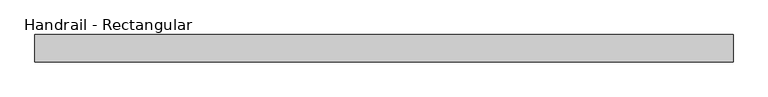
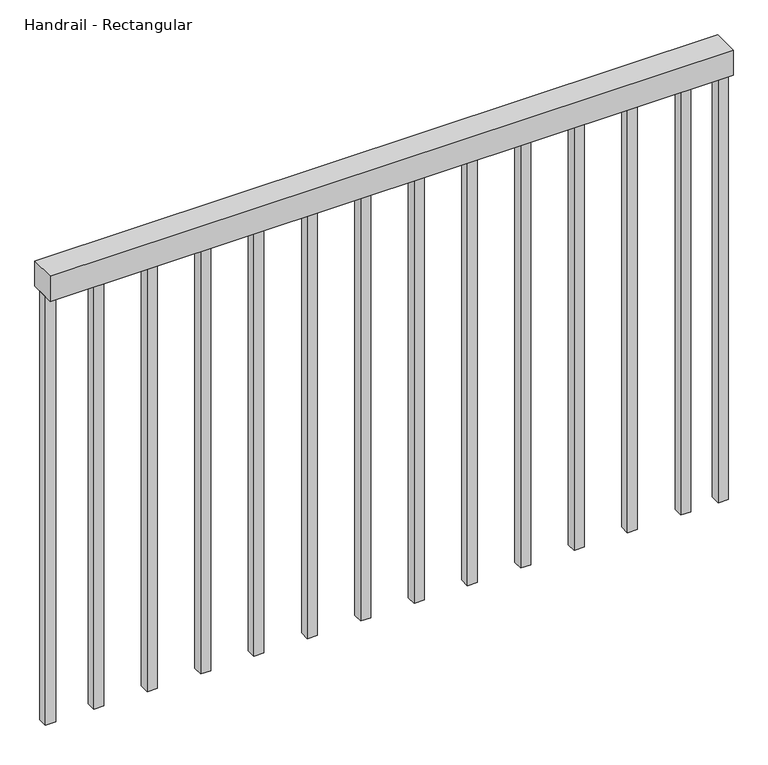
"""IFC4 building model written with IfcOpenShell, lengths in millimetres: railing geometry, Handrail - Rectangular."""

from ifc_helpers import new_model, si_unit, frame, origin, place, context, project, spatial, polyline, outline, extrude, source, transform, mapped, element, save


def handrail_rectangular_695a3284(model_context):
    return source(origin(), model_context, "Body", "SweptSolid", [
        extrude(outline(polyline([(-5985.2211091, 9945.0507146), (-5985.2211091, 9995.8507146), (-4685.2211091, 9995.8507146), (-4685.2211091, 9945.0507146), (-5985.2211091, 9945.0507146)])), frame((0.0, 0.0, 6654.4), z_axis=(0.0, 0.0, 1.0), x_axis=(1.0, 0.0, 0.0)), (0.0, 0.0, 1.0), 50.8),
        extrude(outline(polyline([(-4775.5461091, 9960.9257146), (-4775.5461091, 9979.9757146), (-4756.4961091, 9979.9757146), (-4756.4961091, 9960.9257146), (-4775.5461091, 9960.9257146)])), frame((0.0, 0.0, 5790.8), z_axis=(0.0, 0.0, 1.0), x_axis=(1.0, 0.0, 0.0)), (0.0, 0.0, 1.0), 863.6),
        extrude(outline(polyline([(-4877.1461091, 9960.9257146), (-4877.1461091, 9979.9757146), (-4858.0961091, 9979.9757146), (-4858.0961091, 9960.9257146), (-4877.1461091, 9960.9257146)])), frame((0.0, 0.0, 5790.8), z_axis=(0.0, 0.0, 1.0), x_axis=(1.0, 0.0, 0.0)), (0.0, 0.0, 1.0), 863.6),
        extrude(outline(polyline([(-4978.7461091, 9960.9257146), (-4978.7461091, 9979.9757146), (-4959.6961091, 9979.9757146), (-4959.6961091, 9960.9257146), (-4978.7461091, 9960.9257146)])), frame((0.0, 0.0, 5790.8), z_axis=(0.0, 0.0, 1.0), x_axis=(1.0, 0.0, 0.0)), (0.0, 0.0, 1.0), 863.6),
        extrude(outline(polyline([(-5080.3461091, 9960.9257146), (-5080.3461091, 9979.9757146), (-5061.2961091, 9979.9757146), (-5061.2961091, 9960.9257146), (-5080.3461091, 9960.9257146)])), frame((0.0, 0.0, 5790.8), z_axis=(0.0, 0.0, 1.0), x_axis=(1.0, 0.0, 0.0)), (0.0, 0.0, 1.0), 863.6),
        extrude(outline(polyline([(-5181.9461091, 9960.9257146), (-5181.9461091, 9979.9757146), (-5162.8961091, 9979.9757146), (-5162.8961091, 9960.9257146), (-5181.9461091, 9960.9257146)])), frame((0.0, 0.0, 5790.8), z_axis=(0.0, 0.0, 1.0), x_axis=(1.0, 0.0, 0.0)), (0.0, 0.0, 1.0), 863.6),
        extrude(outline(polyline([(-5283.5461091, 9960.9257146), (-5283.5461091, 9979.9757146), (-5264.4961091, 9979.9757146), (-5264.4961091, 9960.9257146), (-5283.5461091, 9960.9257146)])), frame((0.0, 0.0, 5790.8), z_axis=(0.0, 0.0, 1.0), x_axis=(1.0, 0.0, 0.0)), (0.0, 0.0, 1.0), 863.6),
        extrude(outline(polyline([(-5385.1461091, 9960.9257146), (-5385.1461091, 9979.9757146), (-5366.0961091, 9979.9757146), (-5366.0961091, 9960.9257146), (-5385.1461091, 9960.9257146)])), frame((0.0, 0.0, 5790.8), z_axis=(0.0, 0.0, 1.0), x_axis=(1.0, 0.0, 0.0)), (0.0, 0.0, 1.0), 863.6),
        extrude(outline(polyline([(-5486.7461091, 9960.9257146), (-5486.7461091, 9979.9757146), (-5467.6961091, 9979.9757146), (-5467.6961091, 9960.9257146), (-5486.7461091, 9960.9257146)])), frame((0.0, 0.0, 5790.8), z_axis=(0.0, 0.0, 1.0), x_axis=(1.0, 0.0, 0.0)), (0.0, 0.0, 1.0), 863.6),
        extrude(outline(polyline([(-5588.3461091, 9960.9257146), (-5588.3461091, 9979.9757146), (-5569.2961091, 9979.9757146), (-5569.2961091, 9960.9257146), (-5588.3461091, 9960.9257146)])), frame((0.0, 0.0, 5790.8), z_axis=(0.0, 0.0, 1.0), x_axis=(1.0, 0.0, 0.0)), (0.0, 0.0, 1.0), 863.6),
        extrude(outline(polyline([(-5689.9461091, 9960.9257146), (-5689.9461091, 9979.9757146), (-5670.8961091, 9979.9757146), (-5670.8961091, 9960.9257146), (-5689.9461091, 9960.9257146)])), frame((0.0, 0.0, 5790.8), z_axis=(0.0, 0.0, 1.0), x_axis=(1.0, 0.0, 0.0)), (0.0, 0.0, 1.0), 863.6),
        extrude(outline(polyline([(-5791.5461091, 9960.9257146), (-5791.5461091, 9979.9757146), (-5772.4961091, 9979.9757146), (-5772.4961091, 9960.9257146), (-5791.5461091, 9960.9257146)])), frame((0.0, 0.0, 5790.8), z_axis=(0.0, 0.0, 1.0), x_axis=(1.0, 0.0, 0.0)), (0.0, 0.0, 1.0), 863.6),
        extrude(outline(polyline([(-5893.1461091, 9960.9257146), (-5893.1461091, 9979.9757146), (-5874.0961091, 9979.9757146), (-5874.0961091, 9960.9257146), (-5893.1461091, 9960.9257146)])), frame((0.0, 0.0, 5790.8), z_axis=(0.0, 0.0, 1.0), x_axis=(1.0, 0.0, 0.0)), (0.0, 0.0, 1.0), 863.6),
        extrude(outline(polyline([(-4704.2711091, 9960.9257146), (-4704.2711091, 9979.9757146), (-4685.2211091, 9979.9757146), (-4685.2211091, 9960.9257146), (-4704.2711091, 9960.9257146)])), frame((0.0, 0.0, 5790.8), z_axis=(0.0, 0.0, 1.0), x_axis=(1.0, 0.0, 0.0)), (0.0, 0.0, 1.0), 863.6),
        extrude(outline(polyline([(-5985.2211091, 9960.9257146), (-5985.2211091, 9979.9757146), (-5966.1711091, 9979.9757146), (-5966.1711091, 9960.9257146), (-5985.2211091, 9960.9257146)])), frame((0.0, 0.0, 5790.8), z_axis=(0.0, 0.0, 1.0), x_axis=(1.0, 0.0, 0.0)), (0.0, 0.0, 1.0), 863.6),
    ])


if __name__ == "__main__":
    model = new_model("IFC4")
    model_context = context("Model", 3, world=origin())
    ifc_project = project(units=[si_unit("LENGTHUNIT", "METRE", prefix="MILLI")], contexts=[model_context])
    site = spatial("IfcSite", under=ifc_project)
    building = spatial("IfcBuilding", under=site)
    placement = place(None, origin())
    handrail_rectangular_shape = handrail_rectangular_695a3284(model_context)
    element("IfcRailing", 1, ObjectType="Handrail - Rectangular", at=placement, inside=building, context=model_context, shape_type="MappedRepresentation", body=[
        mapped(handrail_rectangular_shape, transform((0.0, 0.0, 0.0), x_axis=(1.0, 0.0, 0.0), y_axis=(0.0, 1.0, 0.0), z_axis=(0.0, 0.0, 1.0))),
    ])
    save(model, "model.ifc")
